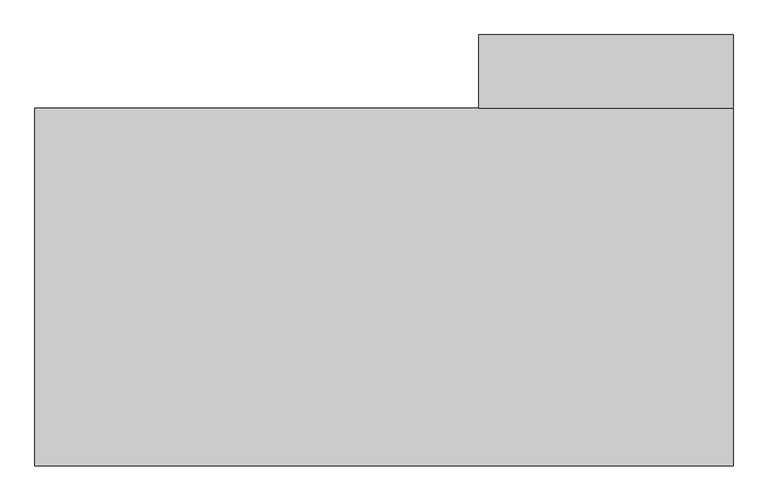
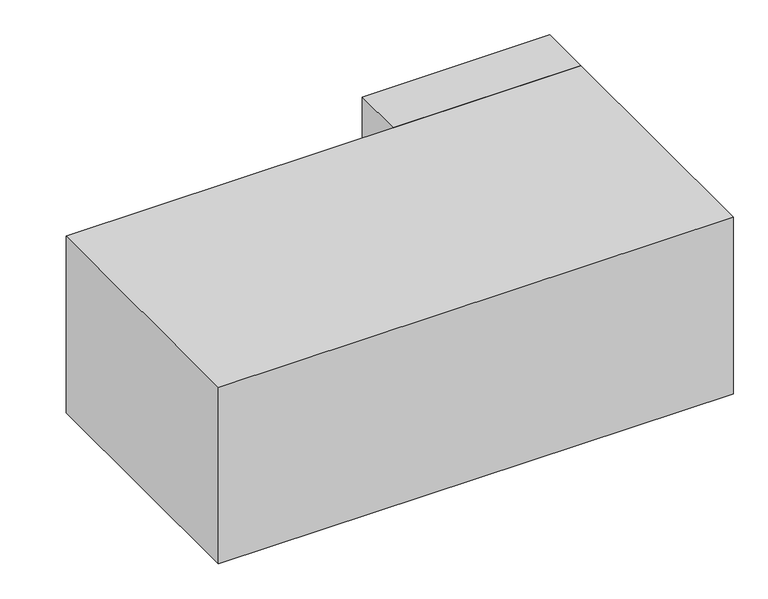
"""IFC4 building model written with IfcOpenShell, lengths in millimetres: proxy geometry, Trane - 20-75 Ton Packaged Ind Rooftop DX Cooling Only and Extended Casing TAG(SXHLF20) 0210035350 : SXHLF20."""

from ifc_helpers import new_model, si_unit, point, frame, frame_2d, origin, origin_with_axes, place, context, project, spatial, polyline, circle_curve, trimmed, segment, composite_curve, outline, extrude, source, transform, mapped, element, save


def mechanical_equipment_7dcddeb3(model_context):
    return source(origin(), model_context, "Body", "SweptSolid", [
        extrude(outline(polyline([(9764.7125, 4713.2875), (9764.7125, 3494.0875), (5529.2625, 3494.0875), (5529.2625, 4713.2875), (9764.7125, 4713.2875)])), origin_with_axes(), (0.0, 0.0, 1.0), 4221.1625),
        extrude(outline(polyline([(9763.91875, 3494.0875), (9763.91875, -2465.3875), (-1858.16875, -2465.3875), (-1858.16875, 3494.0875), (9763.91875, 3494.0875)])), origin_with_axes(), (0.0, 0.0, 1.0), 4221.1625),
        extrude(outline(polyline([(701.548, -26.162), (701.548, 0.0), (7298.944, 0.0), (7298.944, 2247.9), (701.548, 2247.9), (701.548, 2274.062), (7324.598, 2274.062), (7324.598, -26.162), (701.548, -26.162)])), frame((0.0, 0.0, 91.44), z_axis=(0.0, 0.0, 1.0), x_axis=(1.0, 0.0, 0.0)), (0.0, 0.0, 1.0), 25.4),
        extrude(outline(polyline([(7298.944, 0.0), (0.0, 0.0), (0.0, 2247.9), (7298.944, 2247.9), (7298.944, 0.0)]), holes=[polyline([(121.92, 121.92), (7177.024, 121.92), (7177.024, 2125.98), (121.92, 2125.98), (121.92, 121.92)])]), origin_with_axes(), (0.0, 0.0, 1.0), 116.84),
        extrude(outline(polyline([(120.4977028, 1147.0005), (2125.5102028, 1147.0005), (2125.5102028, 121.4755), (120.4977028, 121.4755), (120.4977028, 1147.0005)])), frame((0.0, 0.0, 116.84), z_axis=(0.0, 0.0, 1.0), x_axis=(1.0, 0.0, 0.0)), (0.0, 0.0, 1.0), 25.4),
        extrude(outline(polyline([(5621.1852028, 2125.98), (5621.1852028, 424.18), (4948.0852028, 424.18), (4948.0852028, 2125.98), (5621.1852028, 2125.98)])), frame((0.0, 0.0, 116.84), z_axis=(0.0, 0.0, 1.0), x_axis=(1.0, 0.0, 0.0)), (0.0, 0.0, 1.0), 25.4),
        extrude(outline(polyline([(-0.9777972, 2247.9), (-0.9777972, 0.0), (701.548, 0.0), (701.548, -26.162), (-27.1397972, -26.162), (-27.1397972, 2274.062), (701.548, 2274.062), (701.548, 2247.9), (-0.9777972, 2247.9)])), frame((0.0, 0.0, 91.44), z_axis=(0.0, 0.0, 1.0), x_axis=(1.0, 0.0, 0.0)), (0.0, 0.0, 1.0), 25.4),
        extrude(outline(polyline([(5772.6072, -26.162), (-26.67, -26.162), (-26.67, 2274.062), (5772.6072, 2274.062), (5772.6072, -26.162)])), frame((0.0, 0.0, 116.84), z_axis=(0.0, 0.0, 1.0), x_axis=(1.0, 0.0, 0.0)), (0.0, 0.0, 1.0), 1033.78),
        extrude(outline(composite_curve([segment(trimmed(circle_curve(frame_2d((6534.6035682, 714.4686845)), 355.4662335), [point((6179.1373347, 714.4686845))], [point((6890.0698018, 714.4686845))], False, "CARTESIAN"), True, "CONTINUOUS"), segment(trimmed(circle_curve(frame_2d((6534.6035682, 714.4686845)), 355.4662335), [point((6890.0698018, 714.4686845))], [point((6179.1373347, 714.4686845))], False, "CARTESIAN"), True, "CONTINUOUS")], self_intersect=False)), frame((0.0, 0.0, 2057.4), z_axis=(0.0, 0.0, 1.0), x_axis=(1.0, 0.0, 0.0)), (0.0, 0.0, 1.0), 157.48),
        extrude(outline(composite_curve([segment(trimmed(circle_curve(frame_2d((6534.6044744, 1785.8391493)), 355.4662335), [point((6179.1382408, 1785.8391493))], [point((6890.0707079, 1785.8391493))], False, "CARTESIAN"), True, "CONTINUOUS"), segment(trimmed(circle_curve(frame_2d((6534.6044744, 1785.8391493)), 355.4662335), [point((6890.0707079, 1785.8391493))], [point((6179.1382408, 1785.8391493))], False, "CARTESIAN"), True, "CONTINUOUS")], self_intersect=False)), frame((0.0, 0.0, 2057.4), z_axis=(0.0, 0.0, 1.0), x_axis=(1.0, 0.0, 0.0)), (0.0, 0.0, 1.0), 157.48),
        extrude(outline(polyline([(7298.9601441, 2247.9159493), (7298.9601441, -3.6416507), (5771.3025441, -3.6416507), (5771.3025441, 2247.9159493), (7298.9601441, 2247.9159493)])), frame((0.0, 0.0, 116.84), z_axis=(0.0, 0.0, 1.0), x_axis=(1.0, 0.0, 0.0)), (0.0, 0.0, 1.0), 1940.56),
    ])


if __name__ == "__main__":
    model = new_model("IFC4")
    model_context = context("Model", 3, world=origin())
    ifc_project = project(units=[si_unit("LENGTHUNIT", "METRE", prefix="MILLI")], contexts=[model_context])
    site = spatial("IfcSite", under=ifc_project)
    building = spatial("IfcBuilding", under=site)
    placement = place(None, origin())
    mechanical_equipment_shape = mechanical_equipment_7dcddeb3(model_context)
    element("IfcBuildingElementProxy", 1, Name="Trane - 20-75 Ton Packaged Ind Rooftop DX Cooling Only and Extended Casing TAG(SXHLF20) 0210035350 : SXHLF20", ObjectType="Trane - 20-75 Ton Packaged Ind Rooftop DX Cooling Only and Extended Casing TAG(SXHLF20) 0210035350 : SXHLF20", at=placement, inside=building, context=model_context, shape_type="MappedRepresentation", body=[
        mapped(mechanical_equipment_shape, transform((0.0, 0.0, 0.0), x_axis=(1.0, 0.0, 0.0), y_axis=(0.0, 1.0, 0.0), z_axis=(0.0, 0.0, 1.0))),
    ])
    save(model, "model.ifc")

# Revit data of these elements
# Type "Trane - 20-75 Ton Packaged Ind Rooftop DX Cooling Only and Extended Casing TAG(SXHLF20) 0210035350 : SXHLF20"
#   TAG = "SXHLF20"
#   Serial Number [instance default] = ""
#   Revision = "295"
#   Product URL = "http://www.trane.com/COMMERCIAL/DNA/View.aspx?i=1102"
#   Notes [instance default] = ""
#   Model = "SXHLF204"
#   Manufacturer = "Trane"
#   Literature URL = "http://www.trane.com/Commercial/LiteratureSearchList.aspx?model=SAHL"
#   Equipment Served [instance default] = ""
#   Designation = "RTU"
#   Voltage [instance default] = 460 V
#   Phase [instance default] = 3
#   Frequency [instance default] = 60 Hz
#   Cooling Entering Wet Bulb Temperature = 67 °F
#   Cooling Entering Dry Bulb Temperature = 80 °F
#   CB2Y = 21' - 9 9/16"
#   CB2X = 33' - 5 1/16"
#   CB1Y = 10' - 0 1/4"
#   CB1X = 21' - 3 5/8"
#   Ambient Air Temperature = 95 °F
#   ShowClearances [instance default] = yes
# Element 1 (IfcBuildingElementProxy, "Trane - 20-75 Ton Packaged Ind Rooftop DX Cooling Only and Extended Casing TAG(SXHLF20) 0210035350 : SXHLF20")
#   Materials on its faces: "Clearance"
# Materials
#   "Clearance": class "Unassigned", colour RGB 255 0 0, transparency 0.8, Comments = "Rendering appearance not upgraded "
